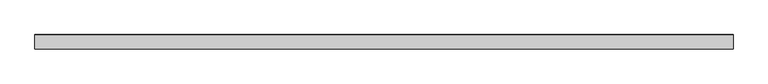
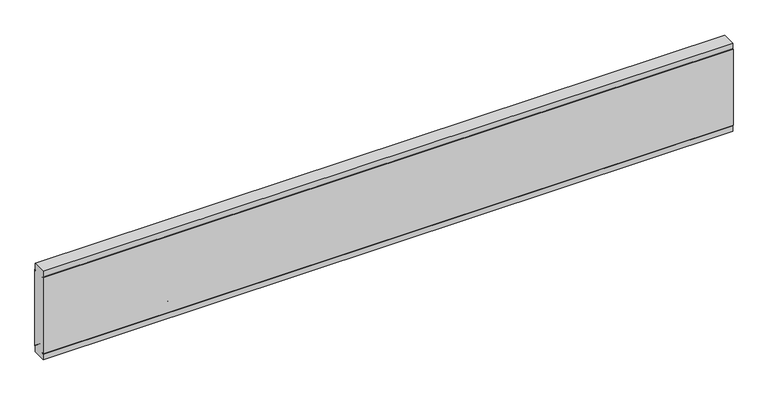
"""IFC4 building model written with IfcOpenShell, lengths in millimetres: proxy geometry, Generic Models 7:Generic Models 1:5:Generic Models 1:5 : Generic Models 7:Generic Models 1:337419:8 : Generic Models 7:Generic Models 1:5:Generic Models 1:5 : Generic Models 7:Generic Models 1:337419:311462."""

from ifc_helpers import new_model, si_unit, origin, place, context, project, spatial, faceted_brep, source, transform, mapped, element, save


def generic_models_e1f4247a(model_context):
    return source(origin(), model_context, "Body", "Brep", [
        faceted_brep([(570490.7367239, -578999.1038841, 4893.9308169), (570490.7367239, -578999.1038841, 3767.0723081), (570490.7367239, -578985.9025672, 3778.1495282), (570490.7367239, -578982.0759722, 3773.5891699), (570490.7367239, -578996.3257591, 3761.632179), (570490.7367239, -578996.3257591, 3679.428125), (570490.7367239, -578801.8570091, 3679.428125), (570490.7367239, -578801.8570091, 3761.632179), (570490.7367239, -578816.1067959, 3773.5891699), (570490.7367239, -578812.2802009, 3778.1495282), (570490.7367239, -578799.0788841, 3767.0723081), (570490.7367239, -578799.0788841, 4092.1340469), (570490.7367239, -578800.666382, 4092.1340469), (570490.7367239, -578800.666382, 4371.7764764), (570490.7367239, -578799.0788841, 4371.7764764), (570490.7367239, -578799.0788841, 4893.9308169), (570490.7367239, -578812.2802009, 4882.8535968), (570490.7367239, -578816.1067959, 4887.4139551), (570490.7367239, -578801.8570091, 4899.370946), (570490.7367239, -578801.8570091, 4981.575), (570490.7367239, -578996.3257591, 4981.575), (570490.7367239, -578996.3257591, 4899.370946), (570490.7367239, -578982.0759722, 4887.4139551), (570490.7367239, -578985.9025672, 4882.8535968), (560859.6126799, -578812.2802009, 3778.1495282), (560859.6126799, -578816.1067959, 3773.5891699), (560859.6126799, -578801.8570091, 3761.632179), (560859.6126799, -578801.8570091, 3679.428125), (560859.6126799, -578996.3257591, 3679.428125), (560859.6126799, -578996.3257591, 3761.632179), (560859.6126799, -578982.0759722, 3773.5891699), (560859.6126799, -578985.9025672, 3778.1495282), (560859.6126799, -578999.1038841, 3767.0723081), (560859.6126799, -578999.1038841, 4893.9308169), (560859.6126799, -578985.9025672, 4882.8535968), (560859.6126799, -578982.0759722, 4887.4139551), (560859.6126799, -578996.3257591, 4899.370946), (560859.6126799, -578996.3257591, 4981.575), (560859.6126799, -578801.8570091, 4981.575), (560859.6126799, -578801.8570091, 4899.370946), (560859.6126799, -578816.1067959, 4887.4139551), (560859.6126799, -578812.2802009, 4882.8535968), (560859.6126799, -578799.0788841, 4893.9308169), (560859.6126799, -578799.0788841, 3970.4796413), (560859.6126799, -578800.666382, 3970.4796413), (560859.6126799, -578800.666382, 3768.404377), (562721.2246473, -578800.666382, 3768.404377), (562689.2549932, -578799.0788841, 3767.0723081), (569873.2872899, -578800.666382, 4320.6273776), (569872.2298741, -578800.666382, 4346.0053577), (569786.7341423, -578800.666382, 4342.4430355), (569787.7915582, -578800.666382, 4317.0650555), (569872.2298741, -578799.0788841, 4346.0053577), (569873.2872899, -578799.0788841, 4320.6273776), (569787.7915582, -578799.0788841, 4317.0650555), (569786.7341423, -578799.0788841, 4342.4430355)], [[[0, 1, 2, 3, 4, 5, 6, 7, 8, 9, 10, 11, 12, 13, 14, 15, 16, 17, 18, 19, 20, 21, 22, 23]], [[24, 25, 26, 27, 28, 29, 30, 31, 32, 33, 34, 35, 36, 37, 38, 39, 40, 41, 42, 43, 44, 45]], [[1, 0, 33, 32]], [[2, 1, 32, 31]], [[3, 2, 31, 30]], [[4, 3, 30, 29]], [[5, 4, 29, 28]], [[6, 5, 28, 27]], [[7, 6, 27, 26]], [[8, 7, 26, 25]], [[9, 8, 25, 24]], [[10, 9, 24, 45, 46, 47]], [[11, 10, 47]], [[16, 15, 42, 41]], [[17, 16, 41, 40]], [[18, 17, 40, 39]], [[19, 18, 39, 38]], [[20, 19, 38, 37]], [[21, 20, 37, 36]], [[22, 21, 36, 35]], [[23, 22, 35, 34]], [[0, 23, 34, 33]], [[48, 49, 13, 12, 46, 45, 44, 50, 51]], [[42, 15, 14, 52, 53, 54, 55, 43]], [[50, 44, 43, 55]], [[51, 50, 55, 54]], [[48, 51, 54, 53]], [[49, 48, 53, 52]], [[46, 12, 11, 47]], [[13, 49, 52, 14]]]),
    ])


if __name__ == "__main__":
    model = new_model("IFC4")
    model_context = context("Model", 3, world=origin())
    ifc_project = project(units=[si_unit("LENGTHUNIT", "METRE", prefix="MILLI")], contexts=[model_context])
    site = spatial("IfcSite", under=ifc_project)
    building = spatial("IfcBuilding", under=site)
    placement = place(None, origin())
    generic_models_shape = generic_models_e1f4247a(model_context)
    element("IfcBuildingElementProxy", 1, Name="Generic Models 7:Generic Models 1:5:Generic Models 1:5 : Generic Models 7:Generic Models 1:337419:8 : Generic Models 7:Generic Models 1:5:Generic Models 1:5 : Generic Models 7:Generic Models 1:337419:311462", ObjectType="Generic Models 7:Generic Models 1:5:Generic Models 1:5 : Generic Models 7:Generic Models 1:337419:8 : Generic Models 7:Generic Models 1:5:Generic Models 1:5 : Generic Models 7:Generic Models 1:337419:311462", at=placement, inside=building, context=model_context, shape_type="MappedRepresentation", body=[
        mapped(generic_models_shape, transform((0.0, 0.0, 0.0), x_axis=(1.0, 0.0, 0.0), y_axis=(0.0, 1.0, 0.0), z_axis=(0.0, 0.0, 1.0))),
    ])
    save(model, "model.ifc")

# Revit data of these elements
# Type "Generic Models 7:Generic Models 1:5:Generic Models 1:5 : Generic Models 7:Generic Models 1:337419:8 : Generic Models 7:Generic Models 1:5:Generic Models 1:5 : Generic Models 7:Generic Models 1:337419:311462"
#   NameOverride = "Generic Models 7:Generic Models 1:5:Generic Models 1:5 : Generic Models 7:Generic Models 1:337419:311462"
#   ObjectTypeOverride = "Generic Models 1:5 : Generic Models 7:Generic Models 1:337419"
#   Reference = "Generic Models 1"
#   Tag = "311462"
# Element 1 (IfcBuildingElementProxy, "Generic Models 7:Generic Models 1:5:Generic Models 1:5 : Generic Models 7:Generic Models 1:337419:8 : Generic Models 7:Generic Models 1:5:Generic Models 1:5 : Generic Models 7:Generic Models 1:337419:311462")
#   Materials on its faces: "FULL CAVITY CLASS A FIBERGLASS INSULATION WITH DURABLE VAPOR BARRIER (BLACK) LINER"
# Materials
#   "FULL CAVITY CLASS A FIBERGLASS INSULATION WITH DURABLE VAPOR BARRIER (BLACK) LINER": class "Unassigned", colour RGB 158 92 175, transparency 0, Cost = 0
